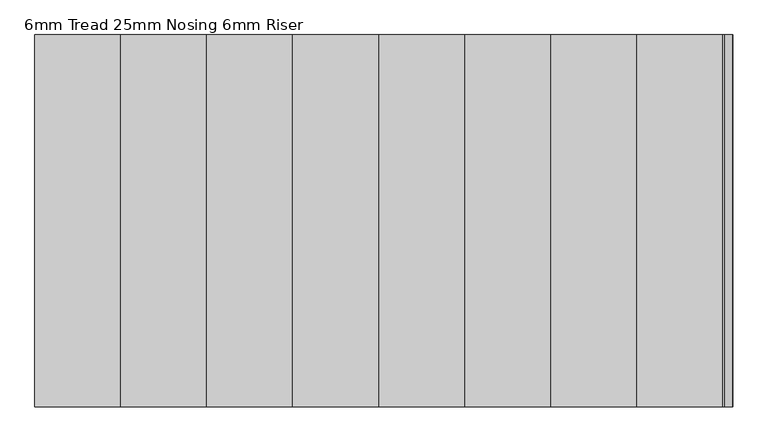
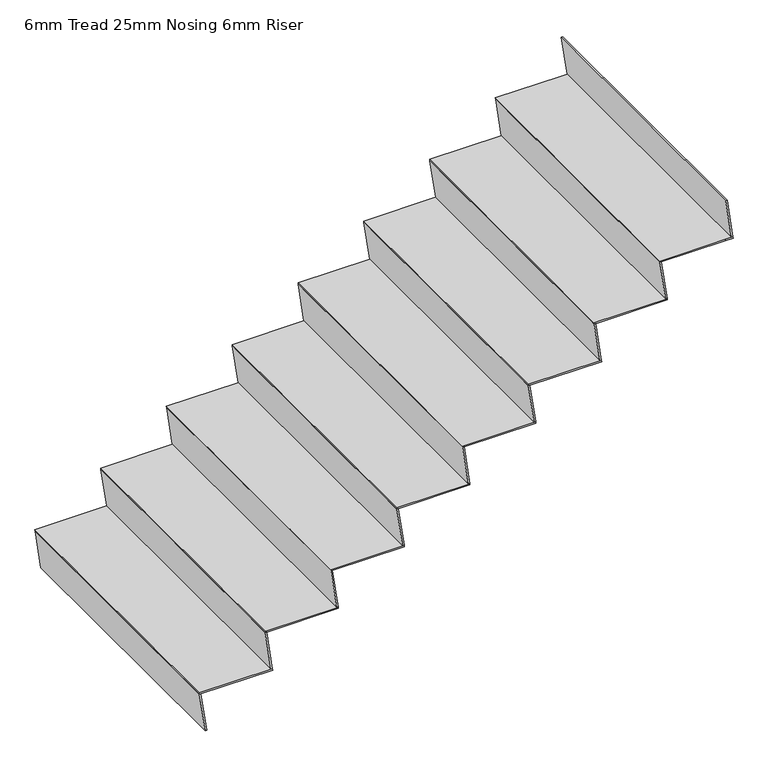
"""IFC4 building model written with IfcOpenShell, lengths in millimetres: stair flight geometry, 6mm Tread 25mm Nosing 6mm Riser."""

from ifc_helpers import new_model, si_unit, origin, place, context, project, spatial, faceted_brep, source, transform, mapped, element, save


def stair_flight_6mm_tread_25mm_nosing_6mm_riser_81022fcb(model_context):
    return source(origin(), model_context, "Body", "Brep", [
        faceted_brep([(-16043.9400908, 12030.4345331, 18588.2352941), (-16043.0900908, 12030.4345331, 18582.2352941), (-16043.0900908, 13220.4345331, 18582.2352941), (-16043.9400908, 13220.4345331, 18588.2352941), (-16350.0, 13220.4345331, 18588.2352941), (-16350.0, 12030.4345331, 18588.2352941), (-16349.15, 12030.4345331, 18582.2352941), (-16349.15, 13220.4345331, 18582.2352941)], [[[0, 1, 2, 3]], [[3, 4, 5, 0]], [[2, 1, 6, 7]], [[4, 3, 2, 7]], [[0, 5, 6, 1]], [[5, 4, 7, 6]]]),
        faceted_brep([(-16349.15, 12030.4345331, 18582.2352941), (-16325.0, 12030.4345331, 18411.7647059), (-16318.9400908, 12030.4345331, 18411.7647059), (-16343.0900908, 12030.4345331, 18582.2352941), (-16349.15, 13220.4345331, 18582.2352941), (-16343.0900908, 13220.4345331, 18582.2352941), (-16318.9400908, 13220.4345331, 18411.7647059), (-16325.0, 13220.4345331, 18411.7647059)], [[[0, 1, 2, 3]], [[4, 5, 6, 7]], [[1, 0, 4, 7]], [[2, 1, 7, 6]], [[3, 2, 6, 5]], [[0, 3, 5, 4]]]),
        faceted_brep([(-16074.15, 12030.4345331, 18758.7058824), (-16050.0, 12030.4345331, 18588.2352941), (-16043.9400908, 12030.4345331, 18588.2352941), (-16068.0900908, 12030.4345331, 18758.7058824), (-16074.15, 13220.4345331, 18758.7058824), (-16068.0900908, 13220.4345331, 18758.7058824), (-16043.9400908, 13220.4345331, 18588.2352941), (-16050.0, 13220.4345331, 18588.2352941)], [[[0, 1, 2, 3]], [[4, 5, 6, 7]], [[1, 0, 4, 7]], [[2, 1, 7, 6]], [[3, 2, 6, 5]], [[0, 3, 5, 4]]]),
        faceted_brep([(-15768.9400908, 13220.4345331, 18764.7058824), (-16075.0, 13220.4345331, 18764.7058824), (-16075.0, 12030.4345331, 18764.7058824), (-15768.9400908, 12030.4345331, 18764.7058824), (-15768.0900908, 13220.4345331, 18758.7058824), (-15768.0900908, 12030.4345331, 18758.7058824), (-16074.15, 12030.4345331, 18758.7058824), (-16074.15, 13220.4345331, 18758.7058824)], [[[0, 1, 2, 3]], [[4, 5, 6, 7]], [[1, 0, 4, 7]], [[3, 2, 6, 5]], [[3, 5, 4, 0]], [[2, 1, 7, 6]]]),
        faceted_brep([(-15799.15, 12030.4345331, 18935.1764706), (-15775.0, 12030.4345331, 18764.7058824), (-15768.9400908, 12030.4345331, 18764.7058824), (-15793.0900908, 12030.4345331, 18935.1764706), (-15799.15, 13220.4345331, 18935.1764706), (-15793.0900908, 13220.4345331, 18935.1764706), (-15768.9400908, 13220.4345331, 18764.7058824), (-15775.0, 13220.4345331, 18764.7058824)], [[[0, 1, 2, 3]], [[4, 5, 6, 7]], [[1, 0, 4, 7]], [[2, 1, 7, 6]], [[3, 2, 6, 5]], [[0, 3, 5, 4]]]),
        faceted_brep([(-15493.9400908, 13220.4345331, 18941.1764706), (-15800.0, 13220.4345331, 18941.1764706), (-15800.0, 12030.4345331, 18941.1764706), (-15493.9400908, 12030.4345331, 18941.1764706), (-15493.0900908, 13220.4345331, 18935.1764706), (-15493.0900908, 12030.4345331, 18935.1764706), (-15799.15, 12030.4345331, 18935.1764706), (-15799.15, 13220.4345331, 18935.1764706)], [[[0, 1, 2, 3]], [[4, 5, 6, 7]], [[1, 0, 4, 7]], [[3, 2, 6, 5]], [[3, 5, 4, 0]], [[2, 1, 7, 6]]]),
        faceted_brep([(-15524.15, 12030.4345331, 19111.6470588), (-15500.0, 12030.4345331, 18941.1764706), (-15493.9400908, 12030.4345331, 18941.1764706), (-15518.0900908, 12030.4345331, 19111.6470588), (-15524.15, 13220.4345331, 19111.6470588), (-15518.0900908, 13220.4345331, 19111.6470588), (-15493.9400908, 13220.4345331, 18941.1764706), (-15500.0, 13220.4345331, 18941.1764706)], [[[0, 1, 2, 3]], [[4, 5, 6, 7]], [[1, 0, 4, 7]], [[2, 1, 7, 6]], [[3, 2, 6, 5]], [[0, 3, 5, 4]]]),
        faceted_brep([(-15218.9400908, 13220.4345331, 19117.6470588), (-15525.0, 13220.4345331, 19117.6470588), (-15525.0, 12030.4345331, 19117.6470588), (-15218.9400908, 12030.4345331, 19117.6470588), (-15218.0900908, 13220.4345331, 19111.6470588), (-15218.0900908, 12030.4345331, 19111.6470588), (-15524.15, 12030.4345331, 19111.6470588), (-15524.15, 13220.4345331, 19111.6470588)], [[[0, 1, 2, 3]], [[4, 5, 6, 7]], [[1, 0, 4, 7]], [[3, 2, 6, 5]], [[3, 5, 4, 0]], [[2, 1, 7, 6]]]),
        faceted_brep([(-15249.15, 12030.4345331, 19288.1176471), (-15225.0, 12030.4345331, 19117.6470588), (-15218.9400908, 12030.4345331, 19117.6470588), (-15243.0900908, 12030.4345331, 19288.1176471), (-15249.15, 13220.4345331, 19288.1176471), (-15243.0900908, 13220.4345331, 19288.1176471), (-15218.9400908, 13220.4345331, 19117.6470588), (-15225.0, 13220.4345331, 19117.6470588)], [[[0, 1, 2, 3]], [[4, 5, 6, 7]], [[1, 0, 4, 7]], [[2, 1, 7, 6]], [[3, 2, 6, 5]], [[0, 3, 5, 4]]]),
        faceted_brep([(-14943.9400908, 13220.4345331, 19294.1176471), (-15250.0, 13220.4345331, 19294.1176471), (-15250.0, 12030.4345331, 19294.1176471), (-14943.9400908, 12030.4345331, 19294.1176471), (-14943.0900908, 13220.4345331, 19288.1176471), (-14943.0900908, 12030.4345331, 19288.1176471), (-15249.15, 12030.4345331, 19288.1176471), (-15249.15, 13220.4345331, 19288.1176471)], [[[0, 1, 2, 3]], [[4, 5, 6, 7]], [[1, 0, 4, 7]], [[3, 2, 6, 5]], [[3, 5, 4, 0]], [[2, 1, 7, 6]]]),
        faceted_brep([(-14974.15, 12030.4345331, 19464.5882353), (-14950.0, 12030.4345331, 19294.1176471), (-14943.9400908, 12030.4345331, 19294.1176471), (-14968.0900908, 12030.4345331, 19464.5882353), (-14974.15, 13220.4345331, 19464.5882353), (-14968.0900908, 13220.4345331, 19464.5882353), (-14943.9400908, 13220.4345331, 19294.1176471), (-14950.0, 13220.4345331, 19294.1176471)], [[[0, 1, 2, 3]], [[4, 5, 6, 7]], [[1, 0, 4, 7]], [[2, 1, 7, 6]], [[3, 2, 6, 5]], [[0, 3, 5, 4]]]),
        faceted_brep([(-14668.9400908, 13220.4345331, 19470.5882353), (-14975.0, 13220.4345331, 19470.5882353), (-14975.0, 12030.4345331, 19470.5882353), (-14668.9400908, 12030.4345331, 19470.5882353), (-14668.0900908, 13220.4345331, 19464.5882353), (-14668.0900908, 12030.4345331, 19464.5882353), (-14974.15, 12030.4345331, 19464.5882353), (-14974.15, 13220.4345331, 19464.5882353)], [[[0, 1, 2, 3]], [[4, 5, 6, 7]], [[1, 0, 4, 7]], [[3, 2, 6, 5]], [[3, 5, 4, 0]], [[2, 1, 7, 6]]]),
        faceted_brep([(-14699.15, 12030.4345331, 19641.0588235), (-14675.0, 12030.4345331, 19470.5882353), (-14668.9400908, 12030.4345331, 19470.5882353), (-14693.0900908, 12030.4345331, 19641.0588235), (-14699.15, 13220.4345331, 19641.0588235), (-14693.0900908, 13220.4345331, 19641.0588235), (-14668.9400908, 13220.4345331, 19470.5882353), (-14675.0, 13220.4345331, 19470.5882353)], [[[0, 1, 2, 3]], [[4, 5, 6, 7]], [[1, 0, 4, 7]], [[2, 1, 7, 6]], [[3, 2, 6, 5]], [[0, 3, 5, 4]]]),
        faceted_brep([(-14393.9400908, 13220.4345331, 19647.0588235), (-14700.0, 13220.4345331, 19647.0588235), (-14700.0, 12030.4345331, 19647.0588235), (-14393.9400908, 12030.4345331, 19647.0588235), (-14393.0900908, 13220.4345331, 19641.0588235), (-14393.0900908, 12030.4345331, 19641.0588235), (-14699.15, 12030.4345331, 19641.0588235), (-14699.15, 13220.4345331, 19641.0588235)], [[[0, 1, 2, 3]], [[4, 5, 6, 7]], [[1, 0, 4, 7]], [[3, 2, 6, 5]], [[3, 5, 4, 0]], [[2, 1, 7, 6]]]),
        faceted_brep([(-14149.15, 12030.4345331, 19994.0), (-14125.0, 12030.4345331, 19823.5294118), (-14118.9400908, 12030.4345331, 19823.5294118), (-14143.0900908, 12030.4345331, 19994.0), (-14149.15, 13220.4345331, 19994.0), (-14143.0900908, 13220.4345331, 19994.0), (-14118.9400908, 13220.4345331, 19823.5294118), (-14125.0, 13220.4345331, 19823.5294118)], [[[0, 1, 2, 3]], [[4, 5, 6, 7]], [[1, 0, 4, 7]], [[2, 1, 7, 6]], [[3, 2, 6, 5]], [[0, 3, 5, 4]]]),
        faceted_brep([(-14424.15, 12030.4345331, 19817.5294118), (-14400.0, 12030.4345331, 19647.0588235), (-14393.9400908, 12030.4345331, 19647.0588235), (-14418.0900908, 12030.4345331, 19817.5294118), (-14424.15, 13220.4345331, 19817.5294118), (-14418.0900908, 13220.4345331, 19817.5294118), (-14393.9400908, 13220.4345331, 19647.0588235), (-14400.0, 13220.4345331, 19647.0588235)], [[[0, 1, 2, 3]], [[4, 5, 6, 7]], [[1, 0, 4, 7]], [[2, 1, 7, 6]], [[3, 2, 6, 5]], [[0, 3, 5, 4]]]),
        faceted_brep([(-14118.9400908, 13220.4345331, 19823.5294118), (-14150.0, 13220.4345331, 19823.5294118), (-14425.0, 13220.4345331, 19823.5294118), (-14425.0, 12030.4345331, 19823.5294118), (-14150.0, 12030.4345331, 19823.5294118), (-14118.9400908, 12030.4345331, 19823.5294118), (-14118.0900908, 13220.4345331, 19817.5294118), (-14118.0900908, 12030.4345331, 19817.5294118), (-14150.0, 12030.4345331, 19817.5294118), (-14424.15, 12030.4345331, 19817.5294118), (-14424.15, 13220.4345331, 19817.5294118), (-14150.0, 13220.4345331, 19817.5294118)], [[[0, 1, 2, 3, 4, 5]], [[6, 7, 8, 9, 10, 11]], [[1, 0, 6, 11]], [[2, 1, 11, 10]], [[4, 3, 9, 8]], [[5, 4, 8, 7]], [[5, 7, 6, 0]], [[3, 2, 10, 9]]]),
    ])


if __name__ == "__main__":
    model = new_model("IFC4")
    model_context = context("Model", 3, world=origin())
    ifc_project = project(units=[si_unit("LENGTHUNIT", "METRE", prefix="MILLI")], contexts=[model_context])
    site = spatial("IfcSite", under=ifc_project)
    building = spatial("IfcBuilding", under=site)
    placement = place(None, origin())
    stair_flight_6mm_tread_25mm_nosing_6mm_riser_shape = stair_flight_6mm_tread_25mm_nosing_6mm_riser_81022fcb(model_context)
    element("IfcStairFlight", 1, ObjectType="6mm Tread 25mm Nosing 6mm Riser", at=placement, inside=building, context=model_context, shape_type="MappedRepresentation", body=[
        mapped(stair_flight_6mm_tread_25mm_nosing_6mm_riser_shape, transform((0.0, 0.0, 0.0), x_axis=(1.0, 0.0, 0.0), y_axis=(0.0, 1.0, 0.0), z_axis=(0.0, 0.0, 1.0))),
    ])
    save(model, "model.ifc")

# Revit data of these elements
# Element 1 (IfcStairFlight, "6mm Tread 25mm Nosing 6mm Riser")
#   Materials on its faces: "Steel, Paint Finish, Dark Gray"
# Materials
#   "Steel, Paint Finish, Dark Gray": class "Metal", colour RGB 89 89 89, transparency 0, Description = "Steel, paint finish, dark gray, glossy", Cost = 0
